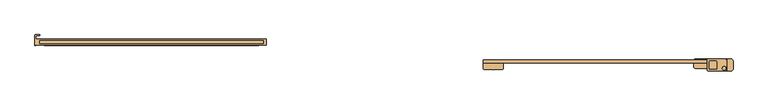
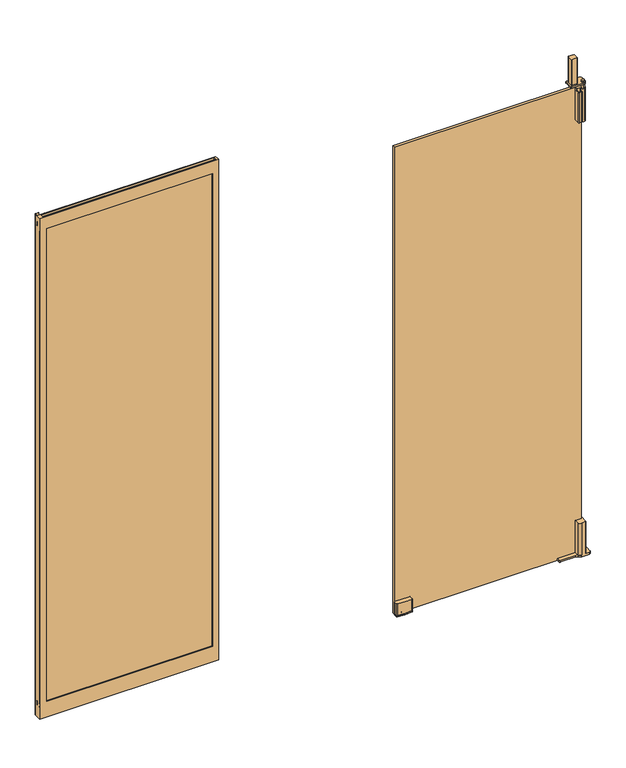
"""IFC4 building model written with IfcOpenShell, lengths in millimetres: door geometry, Otomatik Kapı-Çift Kanat : Otomatik Kapı - Çift Kanat - 150-220."""

from ifc_helpers import new_model, si_unit, frame, origin, origin_with_axes, place, context, project, spatial, polyline, circle_curve, outline, extrude, source, transform, mapped, element, save
from ifc_brep_helpers import plane_surface, cylinder_surface, revolved_surface, advanced_brep


def door_5e92e189(model_context):
    return source(origin(), model_context, "Body", "SolidModel", [
        advanced_brep(
        [(-756.7, 35.2330503, 8.0000212), (-753.7330503, 38.2, 8.0000212), (-741.69925, 38.2, 8.0000212), (-741.69925, 36.2, 8.0000212), (-753.6861454, 36.2, 8.0000212), (-754.7, 35.1861454, 8.0000212), (-754.7, 23.7, 8.0000212), (-2.5, 23.6999918, 8.0000212), (-2.5, 3.7, 8.0000212), (-756.7, 3.7, 8.0000212), (-741.69925, 10.2025832, 8.0000212), (-12.4985, 10.2025832, 8.0000212), (-12.4985, 17.1998167, 8.0000212), (-741.69925, 17.1998167, 8.0000212), (-754.7, 23.7, 2241.0), (-754.7, 35.1861454, 2241.0), (-753.6861454, 36.2, 2241.0), (-741.69925, 36.2, 2241.0), (-741.69925, 38.2, 2241.0), (-753.7330503, 38.2, 2241.0), (-756.7, 35.2330503, 2241.0), (-756.7, 3.7, 2241.0), (-2.5, 3.7, 2241.0), (-2.5, 23.7, 2241.0), (-741.69925, 18.701, 2241.0), (-12.4985, 18.701, 2241.0), (-12.4985, 8.699, 2241.0), (-741.69925, 8.699, 2241.0), (-756.7, 3.7, 78.000055), (-756.7, 5.7, 78.000055), (-756.7, 5.7, 62.9982446), (-756.7, 6.760542, 62.9982446), (-756.7, 6.760542, 2201.0007973), (-756.7, 5.7, 2201.0007973), (-756.7, 5.7, 2186.0007973), (-756.7, 3.7, 2186.0007973), (-726.6862373, 23.7, 2186.0004744), (-726.6862373, 21.7006279, 2186.0004744), (-726.6862373, 21.7006279, 77.9999799), (-726.6862373, 23.7, 77.9999799), (-741.69925, 21.7006279, 2201.0007973), (-741.69925, 21.7006279, 62.9982446), (-12.4985, 21.7006279, 62.9982446), (-12.4985, 21.7006279, 2201.0007973), (-27.4985, 21.7006279, 2186.0004744), (-27.4985, 21.7006279, 77.9999799), (-741.69925, 17.1998167, 33.4998483), (-741.69925, 10.2025832, 33.4998483), (-741.69925, 8.699, 2232.5), (-741.69925, 18.701, 2232.5), (-741.69925, 5.7, 2201.0007973), (-741.69925, 5.7, 62.9982446), (-756.5103756, 5.7, 78.000055), (-756.5103756, 5.7, 62.9982446), (-756.5103756, 5.7, 2201.0007973), (-756.5103756, 5.7, 2186.0007973), (-12.4985, 5.7, 2201.0007973), (-12.4985, 5.7, 62.9982446), (-726.6985, 5.7, 2186.0007973), (-726.6985, 5.7, 78.000055), (-27.4985, 5.7, 78.000055), (-27.4985, 5.7, 2186.0007973), (-726.6985, 3.7, 2186.0007973), (-726.6985, 3.7, 78.000055), (-753.639458, 3.7, 2186.0007973), (-753.639458, 3.7, 78.000055), (-27.4985, 3.7, 2186.0007973), (-27.4985, 3.7, 78.000055), (-27.4985, 23.7, 77.9999799), (-27.4985, 23.7, 2186.0004744), (-12.4985, 8.699, 2232.5), (-12.4985, 18.701, 2232.5), (-12.4985, 17.1998167, 33.4998483), (-12.4985, 10.2025832, 33.4998483)],
        [
            (0, 1, circle_curve(frame((-753.7330503, 35.2330503, 8.0000212), z_axis=(0.0, 0.0, -1.0), x_axis=(-1.0, 0.0, 0.0)), 2.9669497)),
            (1, 2),
            (2, 3),
            (3, 4),
            (4, 5, circle_curve(frame((-753.6861454, 35.1861454, 8.0000212), z_axis=(0.0, 0.0, 1.0), x_axis=(-1.0, 0.0, 0.0)), 1.0138546)),
            (5, 6),
            (6, 7),
            (7, 8),
            (8, 9),
            (9, 0),
            (10, 11),
            (11, 12),
            (12, 13),
            (13, 10),
            (14, 15),
            (15, 16, circle_curve(frame((-753.6861454, 35.1861454, 2241.0), z_axis=(0.0, 0.0, -1.0), x_axis=(-1.0, 0.0, 0.0)), 1.0138546)),
            (16, 17),
            (17, 18),
            (18, 19),
            (19, 20, circle_curve(frame((-753.7330503, 35.2330503, 2241.0), z_axis=(0.0, 0.0, 1.0), x_axis=(-1.0, 0.0, 0.0)), 2.9669497)),
            (20, 21),
            (21, 22),
            (22, 23),
            (23, 14),
            (24, 25),
            (25, 26),
            (26, 27),
            (27, 24),
            (20, 0),
            (9, 28),
            (28, 29),
            (29, 30),
            (30, 31),
            (31, 32),
            (32, 33),
            (33, 34),
            (34, 35),
            (35, 21),
            (1, 19),
            (18, 2),
            (17, 3),
            (36, 37),
            (37, 38),
            (38, 39),
            (39, 36),
            (40, 41),
            (41, 42),
            (42, 43),
            (43, 40),
            (37, 44),
            (44, 45),
            (45, 38),
            (13, 46),
            (46, 47),
            (47, 10),
            (27, 48),
            (48, 49),
            (49, 24),
            (40, 50),
            (50, 51),
            (51, 41),
            (29, 52),
            (52, 53),
            (53, 30),
            (33, 54),
            (54, 55),
            (55, 34),
            (50, 56),
            (56, 57),
            (57, 51),
            (58, 59),
            (59, 60),
            (60, 61),
            (61, 58),
            (58, 62),
            (62, 63),
            (63, 59),
            (35, 64),
            (64, 65),
            (65, 28),
            (8, 22),
            (62, 66),
            (66, 67),
            (67, 63),
            (23, 7),
            (6, 14),
            (39, 68),
            (68, 69),
            (69, 36),
            (16, 4),
            (5, 15),
            (54, 32, circle_curve(frame((-753.639458, 6.760542, 2201.0007973), z_axis=(0.0, 0.0, -1.0), x_axis=(-1.0, 0.0, 0.0)), 3.060542)),
            (31, 53, circle_curve(frame((-753.639458, 6.760542, 62.9982446), z_axis=(0.0, 0.0, 1.0), x_axis=(-1.0, 0.0, 0.0)), 3.060542)),
            (52, 65, circle_curve(frame((-753.639458, 6.760542, 78.000055), z_axis=(0.0, 0.0, 1.0), x_axis=(-1.0, 0.0, 0.0)), 3.060542)),
            (64, 55, circle_curve(frame((-753.639458, 6.760542, 2186.0007973), z_axis=(0.0, 0.0, -1.0), x_axis=(-1.0, 0.0, 0.0)), 3.060542)),
            (26, 70),
            (70, 48),
            (70, 71),
            (71, 49),
            (71, 25),
            (69, 44),
            (43, 56),
            (61, 66),
            (67, 60),
            (57, 42),
            (45, 68),
            (12, 72),
            (72, 46),
            (72, 73),
            (73, 47),
            (73, 11),
        ],
        [
            plane_surface(frame((-756.7, 23.7, 8.0000212), z_axis=(0.0, 0.0, -1.0), x_axis=(0.0, -1.0, 0.0))),
            plane_surface(frame((-756.7, 23.7, 2241.0), z_axis=(0.0, 0.0, 1.0), x_axis=(0.0, -1.0, 0.0))),
            plane_surface(frame((-756.7, 6.760542, 8.0000212), z_axis=(-1.0, 0.0, 0.0), x_axis=(0.0, 0.0, 1.0))),
            plane_surface(frame((-753.7330503, 38.2, 8.0000212), z_axis=(0.0, 1.0, 0.0), x_axis=(0.0, 0.0, 1.0))),
            plane_surface(frame((-741.69925, 38.2, 8.0000212), z_axis=(1.0, 0.0, 0.0), x_axis=(0.0, 0.0, 1.0))),
            plane_surface(frame((-726.6862373, 23.7, 8.0000212), z_axis=(1.0, 0.0, 0.0), x_axis=(0.0, 0.0, 1.0))),
            plane_surface(frame((-726.6862373, 21.7006279, 8.0000212), z_axis=(0.0, -1.0, 0.0), x_axis=(0.0, 0.0, 1.0))),
            plane_surface(frame((-741.69925, 21.7006279, 8.0000212), z_axis=(1.0, 0.0, 0.0), x_axis=(0.0, 0.0, 1.0))),
            plane_surface(frame((-741.69925, 5.7, 8.0000212), z_axis=(0.0, 1.0, 0.0), x_axis=(0.0, 0.0, 1.0))),
            plane_surface(frame((-726.6985, 5.7, 8.0000212), z_axis=(1.0, 0.0, 0.0), x_axis=(0.0, 0.0, 1.0))),
            plane_surface(frame((-726.6985, 3.7, 8.0000212), z_axis=(0.0, -1.0, 0.0), x_axis=(0.0, 0.0, 1.0))),
            plane_surface(frame((-754.7, 23.7, 8.0000212), z_axis=(0.0, 1.0, 0.0), x_axis=(0.0, 0.0, 1.0))),
            plane_surface(frame((-741.69925, 36.2, 8.0000212), z_axis=(0.0, -1.0, 0.0), x_axis=(0.0, 0.0, 1.0))),
            plane_surface(frame((-754.7, 35.1861454, 8.0000212), z_axis=(1.0, 0.0, 0.0), x_axis=(0.0, 0.0, 1.0))),
            cylinder_surface(frame((-753.639458, 6.760542, 8.0000212), z_axis=(0.0, 0.0, -1.0), x_axis=(-1.0, 0.0, 0.0)), 3.060542),
            cylinder_surface(frame((-753.7330503, 35.2330503, 8.0000212), z_axis=(0.0, 0.0, -1.0), x_axis=(-1.0, 0.0, 0.0)), 2.9669497),
            revolved_surface(polyline([(-754.6999999999999, 35.1861454, 2241.0), (-754.6999999999999, 35.1861454, 8.0000212)]), (-753.6861454, 35.1861454, 8.0000212), (0.0, 0.0, 1.0)),
            plane_surface(frame((-2.5, 23.7, 2241.0), z_axis=(1.0, 0.0, 0.0), x_axis=(0.0, -1.0, 0.0))),
            plane_surface(frame((-756.7, 8.699, 2241.0), z_axis=(0.0, 1.0, 0.0), x_axis=(1.0, 0.0, 0.0))),
            plane_surface(frame((-756.7, 8.699, 2232.5), z_axis=(0.0, 0.0, 1.0), x_axis=(1.0, 0.0, 0.0))),
            plane_surface(frame((-756.7, 18.701, 2232.5), z_axis=(0.0, -1.0, 0.0), x_axis=(1.0, 0.0, 0.0))),
            plane_surface(frame((-756.7, 23.7, 2186.0004744), z_axis=(0.0, 0.0, -1.0), x_axis=(1.0, 0.0, 0.0))),
            plane_surface(frame((-756.7, 21.7, 2201.0007973), z_axis=(0.0, 0.0, -1.0), x_axis=(1.0, 0.0, 0.0))),
            plane_surface(frame((-756.7, 5.7, 2186.0007973), z_axis=(0.0, 0.0, -1.0), x_axis=(1.0, 0.0, 0.0))),
            plane_surface(frame((-756.7, 3.7, 78.000055), z_axis=(0.0, 0.0, 1.0), x_axis=(1.0, 0.0, 0.0))),
            plane_surface(frame((-756.7, 5.7, 62.9982446), z_axis=(0.0, 0.0, 1.0), x_axis=(1.0, 0.0, 0.0))),
            plane_surface(frame((-756.7, 21.6999777, 77.9999799), z_axis=(0.0, 0.0, 1.0), x_axis=(1.0, 0.0, 0.0))),
            plane_surface(frame((-756.7, 17.1998167, 8.0000212), z_axis=(0.0, -1.0, 0.0), x_axis=(1.0, 0.0, 0.0))),
            plane_surface(frame((-756.7, 17.1998167, 33.4998483), z_axis=(0.0, 0.0, -1.0), x_axis=(1.0, 0.0, 0.0))),
            plane_surface(frame((-756.7, 10.2025832, 33.4998483), z_axis=(0.0, 1.0, 0.0), x_axis=(1.0, 0.0, 0.0))),
            plane_surface(frame((-27.4985, 3.7, 8.0000212), z_axis=(-1.0, 0.0, 0.0), x_axis=(0.0, 0.0, 1.0))),
            plane_surface(frame((-12.4985, 5.7, 8.0000212), z_axis=(-1.0, 0.0, 0.0), x_axis=(0.0, 0.0, 1.0))),
            plane_surface(frame((-27.4985, 21.7, 8.0000212), z_axis=(-1.0, 0.0, 0.0), x_axis=(0.0, 0.0, 1.0))),
        ],
        [
            (0, [[1, 2, 3, 4, 5, 6, 7, 8, 9, 10], [11, 12, 13, 14]]),
            (1, [[15, 16, 17, 18, 19, 20, 21, 22, 23, 24], [25, 26, 27, 28]]),
            (2, [[29, -10, 30, 31, 32, 33, 34, 35, 36, 37, 38, -21]]),
            (3, [[-2, 39, -19, 40]]),
            (4, [[-3, -40, -18, 41]]),
            (5, [[42, 43, 44, 45]]),
            (6, [[46, 47, 48, 49], [-43, 50, 51, 52]]),
            (7, [[-14, 53, 54, 55]]),
            (7, [[-28, 56, 57, 58]]),
            (7, [[59, 60, 61, -46]]),
            (8, [[-32, 62, 63, 64]]),
            (8, [[-36, 65, 66, 67]]),
            (8, [[-60, 68, 69, 70], [71, 72, 73, 74]]),
            (9, [[75, 76, 77, -71]]),
            (10, [[-22, -38, 78, 79, 80, -30, -9, 81], [82, 83, 84, -76]]),
            (11, [[-24, 85, -7, 86], [87, 88, 89, -45]]),
            (12, [[-4, -41, -17, 90]]),
            (13, [[-6, 91, -15, -86]]),
            (14, [[92, -34, 93, -63, 94, -79, 95, -66]]),
            (15, [[-1, -29, -20, -39]]),
            (16, [[-5, -90, -16, -91]]),
            (17, [[-81, -8, -85, -23]]),
            (18, [[-56, -27, 96, 97]]),
            (19, [[-57, -97, 98, 99]]),
            (20, [[-58, -99, 100, -25]]),
            (21, [[-42, -89, 101, -50]]),
            (22, [[-35, -92, -65]]),
            (22, [[-68, -59, -49, 102]]),
            (23, [[-37, -67, -95, -78]]),
            (23, [[-75, -74, 103, -82]]),
            (24, [[-31, -80, -94, -62]]),
            (24, [[-77, -84, 104, -72]]),
            (25, [[-33, -64, -93]]),
            (25, [[-47, -61, -70, 105]]),
            (26, [[-44, -52, 106, -87]]),
            (27, [[-53, -13, 107, 108]]),
            (28, [[-54, -108, 109, 110]]),
            (29, [[-55, -110, 111, -11]]),
            (30, [[-73, -104, -83, -103]]),
            (31, [[-12, -111, -109, -107]]),
            (31, [[-26, -100, -98, -96]]),
            (31, [[-69, -102, -48, -105]]),
            (32, [[-88, -106, -51, -101]]),
        ],
    ),
        extrude(outline(polyline([(-14.9985, 20.6999853), (-14.9985, 10.7006304), (-738.2, 10.7006304), (-738.2, 20.6999853), (-14.9985, 20.6999853)])), frame((0.0, 0.0, 65.4907153), z_axis=(0.0, 0.0, 1.0), x_axis=(1.0, 0.0, 0.0)), (0.0, 0.0, 1.0), 2133.010082),
        extrude(outline(polyline([(20.6999607, 2198.9584681), (20.6999633, 2215.4578872), (21.6999632, 2215.4578872), (21.6999608, 2200.1996761), (23.2999608, 2200.1994116), (23.2999608, 2199.1856312), (20.6999607, 2198.9584681)])), frame((-756.7, 0.0, 0.0), z_axis=(1.0, 0.0, 0.0), x_axis=(0.0, 1.0, 0.0)), (0.0, 0.0, 1.0), 754.2),
        extrude(outline(polyline([(20.6999853, 79.2411881), (23.2999854, 79.0140251), (23.2999854, 78.0002446), (21.6999855, 77.9999802), (21.6999855, 62.7412326), (20.6999879, 62.7417691), (20.6999853, 79.2411881)])), frame((-756.7, 0.0, 0.0), z_axis=(1.0, 0.0, 0.0), x_axis=(0.0, 1.0, 0.0)), (0.0, 0.0, 1.0), 754.2),
        extrude(outline(polyline([(-737.3860852, 21.7000002), (-726.7, 21.7000002), (-726.7, 23.3000002), (-725.585912, 23.3000002), (-725.2906874, 20.49978), (-737.3860852, 20.49978), (-737.3860852, 21.7000002)])), frame((0.0, 0.0, 8.0000212), z_axis=(0.0, 0.0, 1.0), x_axis=(1.0, 0.0, 0.0)), (0.0, 0.0, 1.0), 2232.9999788),
        advanced_brep(
        [(1467.3535836, -45.0, 150.5), (1493.0, -45.0, 150.5), (1493.0, -54.9832441, 150.5), (1468.0, -54.9832441, 150.5), (1468.0, -73.2159914, 150.5), (1480.406782, -80.0, 150.5), (1498.2162961, -80.0, 150.5), (1500.0, -78.2162961, 150.5), (1500.0, -42.932554, 150.5), (1498.067446, -41.0, 150.5), (1469.2861376, -41.0, 150.5), (1467.3535836, -42.932554, 150.5), (1471.9265924, -76.964766, 8.0), (1468.0, -73.2159914, 8.0), (1470.1692976, -75.2261826, 8.0), (1467.3535836, -45.0, 8.0), (1493.0, -45.0, 8.0), (1493.0, -54.9832441, 8.0), (1468.0, -54.9832441, 8.0), (1480.406782, -80.0, 8.0), (1480.406782, -80.0, 0.0), (1512.8478933, -80.0, 0.0), (1512.8478933, -80.0, 8.0), (1498.2162961, -80.0, 8.0), (1500.0, -78.2162961, 8.0), (1500.0, -42.932554, 8.0), (1498.067446, -41.0, 8.0), (1512.9502869, -41.0, 8.0), (1512.9502869, -41.0, 0.0), (1397.0062198, -41.0, 0.0), (1397.0062198, -41.0, 8.0), (1469.2861376, -41.0, 8.0), (1467.3535836, -42.932554, 8.0), (1520.0062198, -48.0559329, 0.0), (1520.0062198, -72.8416735, 0.0), (1470.1692976, -75.2261826, 0.0), (1461.1062198, -71.0, 0.0), (1397.0062198, -71.0, 0.0), (1392.0062198, -66.0, 0.0), (1392.0062198, -46.0, 0.0), (1520.0062198, -72.8416735, 8.0), (1520.0062198, -48.0559329, 8.0), (1392.0062198, -46.0, 8.0), (1392.0062198, -66.0, 8.0), (1397.0062198, -71.0, 8.0), (1461.1062198, -71.0, 8.0)],
        [
            (0, 1),
            (1, 2),
            (2, 3),
            (3, 4),
            (4, 5, circle_curve(frame((1481.829294, -62.6615339, 150.5), z_axis=(0.0, 0.0, 1.0), x_axis=(-1.0, 0.0, 0.0)), 17.3967223)),
            (5, 6),
            (6, 7, circle_curve(frame((1498.2162961, -78.2162961, 150.5), z_axis=(0.0, 0.0, 1.0), x_axis=(-1.0, 0.0, 0.0)), 1.7837039)),
            (7, 8),
            (8, 9, circle_curve(frame((1498.067446, -42.932554, 150.5), z_axis=(0.0, 0.0, 1.0), x_axis=(-1.0, 0.0, 0.0)), 1.932554)),
            (9, 10),
            (10, 11, circle_curve(frame((1469.2861376, -42.932554, 150.5), z_axis=(0.0, 0.0, 1.0), x_axis=(-1.0, 0.0, 0.0)), 1.932554)),
            (11, 0),
            (12, 13, circle_curve(frame((1481.829294, -62.6615339, 8.0), z_axis=(0.0, 0.0, -1.0), x_axis=(-1.0, 0.0, 0.0)), 17.3967223)),
            (13, 14, circle_curve(frame((1461.1062198, -82.8310079, 8.0), z_axis=(0.0, 0.0, -1.0), x_axis=(-1.0, 0.0, 0.0)), 11.8310079)),
            (14, 12, circle_curve(frame((1480.406782, -66.6359132, 8.0), z_axis=(0.0, 0.0, 1.0), x_axis=(-1.0, 0.0, 0.0)), 13.3640868)),
            (0, 15),
            (15, 16),
            (16, 1),
            (16, 17),
            (17, 2),
            (17, 18),
            (18, 3),
            (18, 13),
            (13, 4),
            (12, 19, circle_curve(frame((1481.829294, -62.6615339, 8.0), z_axis=(0.0, 0.0, 1.0), x_axis=(-1.0, 0.0, 0.0)), 17.3967223)),
            (19, 5),
            (19, 20),
            (20, 21),
            (21, 22),
            (22, 23),
            (23, 6),
            (23, 24, circle_curve(frame((1498.2162961, -78.2162961, 8.0), z_axis=(0.0, 0.0, 1.0), x_axis=(-1.0, 0.0, 0.0)), 1.7837039)),
            (24, 7),
            (24, 25),
            (25, 8),
            (25, 26, circle_curve(frame((1498.067446, -42.932554, 8.0), z_axis=(0.0, 0.0, 1.0), x_axis=(-1.0, 0.0, 0.0)), 1.932554)),
            (26, 9),
            (26, 27),
            (27, 28),
            (28, 29),
            (29, 30),
            (30, 31),
            (31, 10),
            (31, 32, circle_curve(frame((1469.2861376, -42.932554, 8.0), z_axis=(0.0, 0.0, 1.0), x_axis=(-1.0, 0.0, 0.0)), 1.932554)),
            (32, 11),
            (32, 15),
            (28, 33, circle_curve(frame((1512.9502869, -48.0559329, 0.0), z_axis=(0.0, 0.0, -1.0), x_axis=(-1.0, 0.0, 0.0)), 7.0559329)),
            (33, 34),
            (34, 21, circle_curve(frame((1512.8478933, -72.8416735, 0.0), z_axis=(0.0, 0.0, -1.0), x_axis=(-1.0, 0.0, 0.0)), 7.1583265)),
            (20, 35, circle_curve(frame((1480.406782, -66.6359132, 0.0), z_axis=(0.0, 0.0, -1.0), x_axis=(-1.0, 0.0, 0.0)), 13.3640868)),
            (35, 36, circle_curve(frame((1461.1062198, -82.8310079, 0.0), z_axis=(0.0, 0.0, 1.0), x_axis=(-1.0, 0.0, 0.0)), 11.8310079)),
            (36, 37),
            (37, 38, circle_curve(frame((1397.0062198, -66.0, 0.0), z_axis=(0.0, 0.0, -1.0), x_axis=(-1.0, 0.0, 0.0)), 5.0)),
            (38, 39),
            (39, 29, circle_curve(frame((1397.0062198, -46.0, 0.0), z_axis=(0.0, 0.0, -1.0), x_axis=(-1.0, 0.0, 0.0)), 5.0)),
            (12, 19, circle_curve(frame((1480.406782, -66.6359132, 8.0), z_axis=(0.0, 0.0, 1.0), x_axis=(-1.0, 0.0, 0.0)), 13.3640868)),
            (22, 40, circle_curve(frame((1512.8478933, -72.8416735, 8.0), z_axis=(0.0, 0.0, 1.0), x_axis=(-1.0, 0.0, 0.0)), 7.1583265)),
            (40, 41),
            (41, 27, circle_curve(frame((1512.9502869, -48.0559329, 8.0), z_axis=(0.0, 0.0, 1.0), x_axis=(-1.0, 0.0, 0.0)), 7.0559329)),
            (30, 42, circle_curve(frame((1397.0062198, -46.0, 8.0), z_axis=(0.0, 0.0, 1.0), x_axis=(-1.0, 0.0, 0.0)), 5.0)),
            (42, 43),
            (43, 44, circle_curve(frame((1397.0062198, -66.0, 8.0), z_axis=(0.0, 0.0, 1.0), x_axis=(-1.0, 0.0, 0.0)), 5.0)),
            (44, 45),
            (45, 13, circle_curve(frame((1461.1062198, -82.8310079, 8.0), z_axis=(0.0, 0.0, -1.0), x_axis=(-1.0, 0.0, 0.0)), 11.8310079)),
            (41, 33),
            (40, 34),
            (14, 35),
            (45, 36),
            (44, 37),
            (43, 38),
            (42, 39),
        ],
        [
            plane_surface(frame((1520.0062198, -41.0, 150.5), z_axis=(0.0, 0.0, 1.0), x_axis=(0.0, 1.0, 0.0))),
            plane_surface(frame((1520.0062198, -41.0, 8.0), z_axis=(0.0, 0.0, -1.0), x_axis=(0.0, 1.0, 0.0))),
            plane_surface(frame((1467.3535836, -45.0, 150.5), z_axis=(0.0, -1.0, 0.0), x_axis=(0.0, 0.0, -1.0))),
            plane_surface(frame((1493.0, -45.0, 150.5), z_axis=(-1.0, 0.0, 0.0), x_axis=(0.0, 0.0, -1.0))),
            plane_surface(frame((1493.0, -54.9832441, 150.5), z_axis=(0.0, 1.0, 0.0), x_axis=(0.0, 0.0, -1.0))),
            plane_surface(frame((1468.0, -54.9832441, 150.5), z_axis=(-1.0, 0.0, 0.0), x_axis=(0.0, 0.0, -1.0))),
            cylinder_surface(frame((1481.829294, -62.6615339, 150.5), z_axis=(0.0, 0.0, 1.0), x_axis=(-1.0, 0.0, 0.0)), 17.3967223),
            plane_surface(frame((1480.406782, -80.0, 150.5), z_axis=(0.0, -1.0, 0.0), x_axis=(0.0, 0.0, -1.0))),
            cylinder_surface(frame((1498.2162961, -78.2162961, 150.5), z_axis=(0.0, 0.0, 1.0), x_axis=(-1.0, 0.0, 0.0)), 1.7837039),
            plane_surface(frame((1500.0, -78.2162961, 150.5), z_axis=(1.0, 0.0, 0.0), x_axis=(0.0, 0.0, -1.0))),
            cylinder_surface(frame((1498.067446, -42.932554, 150.5), z_axis=(0.0, 0.0, 1.0), x_axis=(-1.0, 0.0, 0.0)), 1.932554),
            plane_surface(frame((1498.067446, -41.0, 150.5), z_axis=(0.0, 1.0, 0.0), x_axis=(0.0, 0.0, -1.0))),
            cylinder_surface(frame((1469.2861376, -42.932554, 150.5), z_axis=(0.0, 0.0, 1.0), x_axis=(-1.0, 0.0, 0.0)), 1.932554),
            plane_surface(frame((1467.3535836, -42.932554, 150.5), z_axis=(-1.0, 0.0, 0.0), x_axis=(0.0, 0.0, -1.0))),
            plane_surface(frame((1520.0062198, -41.0, 0.0), z_axis=(0.0, 0.0, -1.0), x_axis=(0.0, 1.0, 0.0))),
            plane_surface(frame((1520.0062198, -41.0, 8.0), z_axis=(0.0, 0.0, 1.0), x_axis=(0.0, 1.0, 0.0))),
            cylinder_surface(frame((1512.9502869, -48.0559329, 0.0), z_axis=(0.0, 0.0, -1.0), x_axis=(-1.0, 0.0, 0.0)), 7.0559329),
            plane_surface(frame((1520.0062198, -48.0559329, 0.0), z_axis=(1.0, 0.0, 0.0), x_axis=(0.0, 0.0, 1.0))),
            cylinder_surface(frame((1512.8478933, -72.8416735, 0.0), z_axis=(0.0, 0.0, -1.0), x_axis=(-1.0, 0.0, 0.0)), 7.1583265),
            cylinder_surface(frame((1480.406782, -66.6359132, 0.0), z_axis=(0.0, 0.0, -1.0), x_axis=(-1.0, 0.0, 0.0)), 13.3640868),
            revolved_surface(polyline([(1449.2752119, -82.8310079, 8.0), (1449.2752119, -82.8310079, 0.0)]), (1461.1062198, -82.8310079, 0.0), (0.0, 0.0, 1.0)),
            plane_surface(frame((1461.1062198, -71.0, 0.0), z_axis=(0.0, -1.0, 0.0), x_axis=(0.0, 0.0, 1.0))),
            cylinder_surface(frame((1397.0062198, -66.0, 0.0), z_axis=(0.0, 0.0, -1.0), x_axis=(-1.0, 0.0, 0.0)), 5.0),
            plane_surface(frame((1392.0062198, -66.0, 0.0), z_axis=(-1.0, 0.0, 0.0), x_axis=(0.0, 0.0, 1.0))),
            cylinder_surface(frame((1397.0062198, -46.0, 0.0), z_axis=(0.0, 0.0, -1.0), x_axis=(-1.0, 0.0, 0.0)), 5.0),
        ],
        [
            (0, [[1, 2, 3, 4, 5, 6, 7, 8, 9, 10, 11, 12]]),
            (1, [[13, 14, 15]]),
            (2, [[-1, 16, 17, 18]]),
            (3, [[-2, -18, 19, 20]]),
            (4, [[-3, -20, 21, 22]]),
            (5, [[-4, -22, 23, 24]]),
            (6, [[-5, -24, -13, 25, 26]]),
            (7, [[-6, -26, 27, 28, 29, 30, 31]]),
            (8, [[-7, -31, 32, 33]]),
            (9, [[-8, -33, 34, 35]]),
            (10, [[-9, -35, 36, 37]]),
            (11, [[-10, -37, 38, 39, 40, 41, 42, 43]]),
            (12, [[-11, -43, 44, 45]]),
            (13, [[-12, -45, 46, -16]]),
            (14, [[-40, 47, 48, 49, -28, 50, 51, 52, 53, 54, 55]]),
            (15, [[56, -25]]),
            (15, [[57, 58, 59, -38, -36, -34, -32, -30]]),
            (15, [[60, 61, 62, 63, 64, -23, -21, -19, -17, -46, -44, -42]]),
            (16, [[-47, -39, -59, 65]]),
            (17, [[-48, -65, -58, 66]]),
            (18, [[-49, -66, -57, -29]]),
            (19, [[-50, -27, -56, -15, 67]]),
            (20, [[-51, -67, -14, -64, 68]]),
            (21, [[-52, -68, -63, 69]]),
            (22, [[-53, -69, -62, 70]]),
            (23, [[-54, -70, -61, 71]]),
            (24, [[-55, -71, -60, -41]]),
        ],
    ),
        advanced_brep(
        [(1465.150075, -48.2790947, 2225.0), (1443.8206454, -48.2790947, 2225.0), (1441.9853602, -50.1143799, 2225.0), (1441.9853602, -71.4438095, 2225.0), (1443.8206454, -73.2790947, 2225.0), (1465.150075, -73.2790947, 2225.0), (1466.9853602, -71.4438095, 2225.0), (1466.9853602, -50.1143799, 2225.0), (1465.150075, -48.2790947, 2110.0), (1443.8206454, -48.2790947, 2110.0), (1441.9853602, -50.1143799, 2110.0), (1441.9853602, -71.4438095, 2110.0), (1443.8206454, -73.2790947, 2110.0), (1465.150075, -73.2790947, 2110.0), (1466.9853602, -71.4438095, 2110.0), (1466.9853602, -50.1143799, 2110.0), (1439.0026222, -41.0, 2110.0), (1436.0, -44.0026222, 2110.0), (1436.0, -77.6784243, 2110.0), (1439.3215757, -81.0, 2110.0), (1491.0, -81.0, 2110.0), (1500.0, -72.0, 2110.0), (1500.0, -49.8288404, 2110.0), (1491.1711596, -41.0, 2110.0), (1491.0, -77.9, 2110.0), (1491.0, -66.1, 2110.0), (1439.0026222, -41.0, 2104.0), (1491.1711596, -41.0, 2104.0), (1500.0, -49.8288404, 2104.0), (1500.0, -72.0, 2104.0), (1491.0, -81.0, 2104.0), (1439.3215757, -81.0, 2104.0), (1436.0, -77.6784243, 2104.0), (1436.0, -44.0026222, 2104.0), (1491.0, -66.1, 2104.0), (1491.0, -77.9, 2104.0), (1500.0, -72.0, 1938.2), (1484.4524153, -78.1748793, 1938.2), (1480.4177248, -81.0, 1938.2), (1471.1, -81.0, 1938.2), (1468.0, -77.9, 1938.2), (1468.0, -55.1, 1938.2), (1492.8, -55.1, 1938.2), (1492.8, -45.1, 1938.2), (1468.0, -45.1, 1938.2), (1468.0, -42.3259879, 1938.2), (1469.3259879, -41.0, 1938.2), (1498.7883994, -41.0, 1938.2), (1500.0, -42.2116006, 1938.2), (1480.2256421, -66.1, 1938.2), (1471.1, -66.1, 1938.2), (1471.1, -76.9112221, 1938.2), (1472.0887779, -77.9, 1938.2), (1480.1735897, -77.9, 1938.2), (1481.9491878, -75.7274684, 1938.2), (1482.0, -67.8743579, 1938.2), (1491.0, -66.1, 1938.2), (1491.0, -77.9, 1938.2), (1500.0, -72.0, 2083.2), (1500.0, -42.2116006, 2083.2), (1498.7883994, -41.0, 2083.2), (1469.3259879, -41.0, 2083.2), (1468.0, -42.3259879, 2083.2), (1468.0, -45.1, 2083.2), (1492.8, -45.1, 2083.2), (1492.8, -55.1, 2083.2), (1468.0, -55.1, 2083.2), (1468.0, -64.9220198, 2083.2), (1469.1779802, -66.1, 2083.2), (1480.2256421, -66.1, 2083.2), (1482.0, -67.8743579, 2083.2), (1482.0, -72.0, 2083.2), (1491.0, -77.9, 2083.2), (1491.0, -66.1, 2083.2), (1468.0, -77.9, 2073.2), (1468.0, -64.9220198, 2073.2), (1469.1779802, -66.1, 2073.2), (1471.1, -66.1, 2073.2), (1482.0, -75.7274684, 2073.2), (1482.0, -72.0, 2073.2), (1484.4524153, -78.1748793, 2073.2), (1491.0, -77.9, 2083.2), (1491.0, -66.1, 2083.2), (1471.1, -81.0, 2073.2), (1480.4177248, -81.0, 2073.2), (1480.1735897, -77.9, 2073.2), (1472.0887779, -77.9, 2073.2), (1471.1, -76.9112221, 2073.2), (1491.0, -66.1, 2116.5286826), (1491.0, -77.9, 2116.5286826)],
        [
            (0, 1),
            (1, 2, circle_curve(frame((1443.8206454, -50.1143799, 2225.0), z_axis=(0.0, 0.0, 1.0), x_axis=(0.0, -1.0, 0.0)), 1.8352852)),
            (2, 3),
            (3, 4, circle_curve(frame((1443.8206454, -71.4438095, 2225.0), z_axis=(0.0, 0.0, 1.0), x_axis=(0.0, 1.0, 0.0)), 1.8352852)),
            (4, 5),
            (5, 6, circle_curve(frame((1465.150075, -71.4438095, 2225.0), z_axis=(0.0, 0.0, 1.0), x_axis=(0.0, 1.0, 0.0)), 1.8352852)),
            (6, 7),
            (7, 0, circle_curve(frame((1465.150075, -50.1143799, 2225.0), z_axis=(0.0, 0.0, 1.0), x_axis=(0.0, -1.0, 0.0)), 1.8352852)),
            (0, 8),
            (8, 9),
            (9, 1),
            (9, 10, circle_curve(frame((1443.8206454, -50.1143799, 2110.0), z_axis=(0.0, 0.0, 1.0), x_axis=(0.0, -1.0, 0.0)), 1.8352852)),
            (10, 2),
            (10, 11),
            (11, 3),
            (11, 12, circle_curve(frame((1443.8206454, -71.4438095, 2110.0), z_axis=(0.0, 0.0, 1.0), x_axis=(0.0, 1.0, 0.0)), 1.8352852)),
            (12, 4),
            (12, 13),
            (13, 5),
            (13, 14, circle_curve(frame((1465.150075, -71.4438095, 2110.0), z_axis=(0.0, 0.0, 1.0), x_axis=(0.0, 1.0, 0.0)), 1.8352852)),
            (14, 6),
            (14, 15),
            (15, 7),
            (15, 8, circle_curve(frame((1465.150075, -50.1143799, 2110.0), z_axis=(0.0, 0.0, 1.0), x_axis=(0.0, -1.0, 0.0)), 1.8352852)),
            (16, 17, circle_curve(frame((1439.0026222, -44.0026222, 2110.0), z_axis=(0.0, 0.0, 1.0), x_axis=(0.0, -1.0, 0.0)), 3.0026222)),
            (17, 18),
            (18, 19, circle_curve(frame((1439.3215757, -77.6784243, 2110.0), z_axis=(0.0, 0.0, 1.0), x_axis=(0.0, -1.0, 0.0)), 3.3215757)),
            (19, 20),
            (20, 21, circle_curve(frame((1491.0, -72.0, 2110.0), z_axis=(0.0, 0.0, 1.0), x_axis=(0.0, -1.0, 0.0)), 9.0)),
            (21, 22),
            (22, 23, circle_curve(frame((1491.1711596, -49.8288404, 2110.0), z_axis=(0.0, 0.0, 1.0), x_axis=(0.0, -1.0, 0.0)), 8.8288404)),
            (23, 16),
            (24, 25, circle_curve(frame((1491.0, -72.0, 2110.0), z_axis=(0.0, 0.0, -1.0), x_axis=(0.0, -1.0, 0.0)), 5.9)),
            (25, 24, circle_curve(frame((1491.0, -72.0, 2110.0), z_axis=(0.0, 0.0, -1.0), x_axis=(0.0, -1.0, 0.0)), 5.9)),
            (26, 27),
            (27, 28, circle_curve(frame((1491.1711596, -49.8288404, 2104.0), z_axis=(0.0, 0.0, -1.0), x_axis=(0.0, -1.0, 0.0)), 8.8288404)),
            (28, 29),
            (29, 30, circle_curve(frame((1491.0, -72.0, 2104.0), z_axis=(0.0, 0.0, -1.0), x_axis=(0.0, -1.0, 0.0)), 9.0)),
            (30, 31),
            (31, 32, circle_curve(frame((1439.3215757, -77.6784243, 2104.0), z_axis=(0.0, 0.0, -1.0), x_axis=(0.0, -1.0, 0.0)), 3.3215757)),
            (32, 33),
            (33, 26, circle_curve(frame((1439.0026222, -44.0026222, 2104.0), z_axis=(0.0, 0.0, -1.0), x_axis=(0.0, -1.0, 0.0)), 3.0026222)),
            (34, 35, circle_curve(frame((1491.0, -72.0, 2104.0), z_axis=(0.0, 0.0, 1.0), x_axis=(0.0, -1.0, 0.0)), 5.9)),
            (35, 34, circle_curve(frame((1491.0, -72.0, 2104.0), z_axis=(0.0, 0.0, 1.0), x_axis=(0.0, -1.0, 0.0)), 5.9)),
            (23, 27),
            (26, 16),
            (22, 28),
            (21, 29),
            (20, 30),
            (19, 31),
            (18, 32),
            (17, 33),
            (36, 37, circle_curve(frame((1491.0, -72.0, 1938.2), z_axis=(0.0, 0.0, -1.0), x_axis=(0.0, -1.0, 0.0)), 9.0)),
            (37, 38, circle_curve(frame((1479.7322891, -75.7274684, 1938.2), z_axis=(0.0, 0.0, -1.0), x_axis=(0.0, -1.0, 0.0)), 5.3168987)),
            (38, 39),
            (39, 40, circle_curve(frame((1471.1, -77.9, 1938.2), z_axis=(0.0, 0.0, -1.0), x_axis=(0.0, -1.0, 0.0)), 3.1)),
            (40, 41),
            (41, 42),
            (42, 43),
            (43, 44),
            (44, 45),
            (45, 46, circle_curve(frame((1469.3259879, -42.3259879, 1938.2), z_axis=(0.0, 0.0, -1.0), x_axis=(0.0, -1.0, 0.0)), 1.3259879)),
            (46, 47),
            (47, 48, circle_curve(frame((1498.7883994, -42.2116006, 1938.2), z_axis=(0.0, 0.0, -1.0), x_axis=(0.0, -1.0, 0.0)), 1.2116006)),
            (48, 36),
            (49, 50),
            (50, 51),
            (51, 52, circle_curve(frame((1472.0887779, -76.9112221, 1938.2), z_axis=(0.0, 0.0, 1.0), x_axis=(0.0, -1.0, 0.0)), 0.9887779)),
            (52, 53),
            (53, 54, circle_curve(frame((1479.7322891, -75.7274684, 1938.2), z_axis=(0.0, 0.0, 1.0), x_axis=(0.0, -1.0, 0.0)), 2.2168987)),
            (54, 55),
            (55, 49, circle_curve(frame((1480.2256421, -67.8743579, 1938.2), z_axis=(0.0, 0.0, 1.0), x_axis=(0.0, -1.0, 0.0)), 1.7743579)),
            (56, 57, circle_curve(frame((1491.0, -72.0, 1938.2), z_axis=(0.0, 0.0, 1.0), x_axis=(0.0, -1.0, 0.0)), 5.9)),
            (57, 56, circle_curve(frame((1491.0, -72.0, 1938.2), z_axis=(0.0, 0.0, 1.0), x_axis=(0.0, -1.0, 0.0)), 5.9)),
            (58, 59),
            (59, 60, circle_curve(frame((1498.7883994, -42.2116006, 2083.2), z_axis=(0.0, 0.0, 1.0), x_axis=(0.0, -1.0, 0.0)), 1.2116006)),
            (60, 61),
            (61, 62, circle_curve(frame((1469.3259879, -42.3259879, 2083.2), z_axis=(0.0, 0.0, 1.0), x_axis=(0.0, -1.0, 0.0)), 1.3259879)),
            (62, 63),
            (63, 64),
            (64, 65),
            (65, 66),
            (66, 67),
            (67, 68, circle_curve(frame((1469.1779802, -64.9220198, 2083.2), z_axis=(0.0, 0.0, 1.0), x_axis=(0.0, -1.0, 0.0)), 1.1779802)),
            (68, 69),
            (69, 70, circle_curve(frame((1480.2256421, -67.8743579, 2083.2), z_axis=(0.0, 0.0, -1.0), x_axis=(0.0, -1.0, 0.0)), 1.7743579)),
            (70, 71),
            (71, 58, circle_curve(frame((1491.0, -72.0, 2083.2), z_axis=(0.0, 0.0, 1.0), x_axis=(0.0, -1.0, 0.0)), 9.0)),
            (72, 73, circle_curve(frame((1491.0, -72.0, 2083.2), z_axis=(0.0, 0.0, -1.0), x_axis=(0.0, -1.0, 0.0)), 5.9)),
            (73, 72, circle_curve(frame((1491.0, -72.0, 2083.2), z_axis=(0.0, 0.0, -1.0), x_axis=(0.0, -1.0, 0.0)), 5.9)),
            (48, 59),
            (58, 36),
            (47, 60),
            (46, 61),
            (45, 62),
            (44, 63),
            (43, 64),
            (42, 65),
            (41, 66),
            (40, 74),
            (74, 75),
            (75, 67),
            (75, 76, circle_curve(frame((1469.1779802, -64.9220198, 2073.2), z_axis=(0.0, 0.0, 1.0), x_axis=(0.0, -1.0, 0.0)), 1.1779802)),
            (76, 68),
            (76, 77),
            (77, 50),
            (49, 69),
            (55, 70),
            (54, 78),
            (78, 79),
            (79, 71),
            (79, 80, circle_curve(frame((1491.0, -72.0, 2073.2), z_axis=(0.0, 0.0, 1.0), x_axis=(0.0, -1.0, 0.0)), 9.0)),
            (80, 37),
            (57, 81),
            (81, 82, circle_curve(frame((1491.0, -72.0, 2083.2), z_axis=(0.0, 0.0, 1.0), x_axis=(0.0, -1.0, 0.0)), 5.9)),
            (82, 56),
            (82, 81, circle_curve(frame((1491.0, -72.0, 2083.2), z_axis=(0.0, 0.0, 1.0), x_axis=(0.0, -1.0, 0.0)), 5.9)),
            (83, 84),
            (84, 80, circle_curve(frame((1479.7322891, -75.7274684, 2073.2), z_axis=(0.0, 0.0, 1.0), x_axis=(0.0, -1.0, 0.0)), 5.3168987)),
            (78, 85, circle_curve(frame((1479.7322891, -75.7274684, 2073.2), z_axis=(0.0, 0.0, -1.0), x_axis=(0.0, -1.0, 0.0)), 2.2168987)),
            (85, 86),
            (86, 87, circle_curve(frame((1472.0887779, -76.9112221, 2073.2), z_axis=(0.0, 0.0, -1.0), x_axis=(0.0, -1.0, 0.0)), 0.9887779)),
            (87, 77),
            (74, 83, circle_curve(frame((1471.1, -77.9, 2073.2), z_axis=(0.0, 0.0, 1.0), x_axis=(0.0, -1.0, 0.0)), 3.1)),
            (39, 83),
            (87, 51),
            (86, 52),
            (85, 53),
            (84, 38),
            (88, 89, circle_curve(frame((1491.0, -72.0, 2116.5286826), z_axis=(0.0, 0.0, 1.0), x_axis=(0.0, -1.0, 0.0)), 5.9)),
            (89, 88, circle_curve(frame((1491.0, -72.0, 2116.5286826), z_axis=(0.0, 0.0, 1.0), x_axis=(0.0, -1.0, 0.0)), 5.9)),
            (35, 72),
            (73, 34),
            (89, 24),
            (25, 88),
        ],
        [
            plane_surface(frame((1500.0, -41.0, 2225.0), z_axis=(0.0, 0.0, 1.0), x_axis=(1.0, 0.0, 0.0))),
            plane_surface(frame((1465.150075, -48.2790947, 2110.0), z_axis=(0.0, 1.0, 0.0), x_axis=(0.0, 0.0, 1.0))),
            cylinder_surface(frame((1443.8206454, -50.1143799, 2110.0), z_axis=(0.0, 0.0, -1.0), x_axis=(0.0, -1.0, 0.0)), 1.8352852),
            plane_surface(frame((1441.9853602, -50.1143799, 2110.0), z_axis=(-1.0, 0.0, 0.0), x_axis=(0.0, 0.0, 1.0))),
            cylinder_surface(frame((1443.8206454, -71.4438095, 2110.0), z_axis=(0.0, 0.0, -1.0), x_axis=(0.0, 1.0, 0.0)), 1.8352852),
            plane_surface(frame((1443.8206454, -73.2790947, 2110.0), z_axis=(0.0, -1.0, 0.0), x_axis=(0.0, 0.0, 1.0))),
            cylinder_surface(frame((1465.150075, -71.4438095, 2110.0), z_axis=(0.0, 0.0, -1.0), x_axis=(0.0, 1.0, 0.0)), 1.8352852),
            plane_surface(frame((1466.9853602, -71.4438095, 2110.0), z_axis=(1.0, 0.0, 0.0), x_axis=(0.0, 0.0, 1.0))),
            cylinder_surface(frame((1465.150075, -50.1143799, 2110.0), z_axis=(0.0, 0.0, -1.0), x_axis=(0.0, -1.0, 0.0)), 1.8352852),
            plane_surface(frame((1500.0, -41.0, 2110.0), z_axis=(0.0, 0.0, 1.0), x_axis=(1.0, 0.0, 0.0))),
            plane_surface(frame((1500.0, -41.0, 2104.0), z_axis=(0.0, 0.0, -1.0), x_axis=(1.0, 0.0, 0.0))),
            plane_surface(frame((1439.0026222, -41.0, 2110.0), z_axis=(0.0, 1.0, 0.0), x_axis=(0.0, 0.0, -1.0))),
            cylinder_surface(frame((1491.1711596, -49.8288404, 2110.0), z_axis=(0.0, 0.0, 1.0), x_axis=(0.0, -1.0, 0.0)), 8.8288404),
            plane_surface(frame((1500.0, -49.8288404, 2110.0), z_axis=(1.0, 0.0, 0.0), x_axis=(0.0, 0.0, -1.0))),
            cylinder_surface(frame((1491.0, -72.0, 2110.0), z_axis=(0.0, 0.0, 1.0), x_axis=(0.0, -1.0, 0.0)), 9.0),
            plane_surface(frame((1491.0, -81.0, 2110.0), z_axis=(0.0, -1.0, 0.0), x_axis=(0.0, 0.0, -1.0))),
            cylinder_surface(frame((1439.3215757, -77.6784243, 2110.0), z_axis=(0.0, 0.0, 1.0), x_axis=(0.0, -1.0, 0.0)), 3.3215757),
            plane_surface(frame((1436.0, -77.6784243, 2110.0), z_axis=(-1.0, 0.0, 0.0), x_axis=(0.0, 0.0, -1.0))),
            cylinder_surface(frame((1439.0026222, -44.0026222, 2110.0), z_axis=(0.0, 0.0, 1.0), x_axis=(0.0, -1.0, 0.0)), 3.0026222),
            plane_surface(frame((1500.0, -41.0, 1938.2), z_axis=(0.0, 0.0, -1.0), x_axis=(1.0, 0.0, 0.0))),
            plane_surface(frame((1500.0, -41.0, 2083.2), z_axis=(0.0, 0.0, 1.0), x_axis=(1.0, 0.0, 0.0))),
            plane_surface(frame((1500.0, -72.0, 1938.2), z_axis=(1.0, 0.0, 0.0), x_axis=(0.0, 0.0, 1.0))),
            cylinder_surface(frame((1498.7883994, -42.2116006, 1938.2), z_axis=(0.0, 0.0, -1.0), x_axis=(0.0, -1.0, 0.0)), 1.2116006),
            plane_surface(frame((1498.7883994, -41.0, 1938.2), z_axis=(0.0, 1.0, 0.0), x_axis=(0.0, 0.0, 1.0))),
            cylinder_surface(frame((1469.3259879, -42.3259879, 1938.2), z_axis=(0.0, 0.0, -1.0), x_axis=(0.0, -1.0, 0.0)), 1.3259879),
            plane_surface(frame((1468.0, -42.3259879, 1938.2), z_axis=(-1.0, 0.0, 0.0), x_axis=(0.0, 0.0, 1.0))),
            plane_surface(frame((1468.0, -45.1, 1938.2), z_axis=(0.0, -1.0, 0.0), x_axis=(0.0, 0.0, 1.0))),
            plane_surface(frame((1492.8, -45.1, 1938.2), z_axis=(-1.0, 0.0, 0.0), x_axis=(0.0, 0.0, 1.0))),
            plane_surface(frame((1492.8, -55.1, 1938.2), z_axis=(0.0, 1.0, 0.0), x_axis=(0.0, 0.0, 1.0))),
            plane_surface(frame((1468.0, -55.1, 1938.2), z_axis=(-1.0, 0.0, 0.0), x_axis=(0.0, 0.0, 1.0))),
            cylinder_surface(frame((1469.1779802, -64.9220198, 1938.2), z_axis=(0.0, 0.0, -1.0), x_axis=(0.0, -1.0, 0.0)), 1.1779802),
            plane_surface(frame((1469.1779802, -66.1, 1938.2), z_axis=(0.0, -1.0, 0.0), x_axis=(0.0, 0.0, 1.0))),
            revolved_surface(polyline([(1480.2256421, -69.6487158, 2083.2), (1480.2256421, -69.6487158, 1938.2)]), (1480.2256421, -67.8743579, 1938.2), (0.0, 0.0, 1.0)),
            plane_surface(frame((1482.0, -67.8743579, 1938.2), z_axis=(-1.0, 0.0, 0.0), x_axis=(0.0, 0.0, 1.0))),
            cylinder_surface(frame((1491.0, -72.0, 1938.2), z_axis=(0.0, 0.0, -1.0), x_axis=(0.0, -1.0, 0.0)), 9.0),
            revolved_surface(polyline([(1491.0, -77.9, 2083.2), (1491.0, -77.9, 1938.2)]), (1491.0, -72.0, 1938.2), (0.0, 0.0, 1.0)),
            plane_surface(frame((1500.0, -41.0, 2073.2), z_axis=(0.0, 0.0, 1.0), x_axis=(1.0, 0.0, 0.0))),
            cylinder_surface(frame((1471.1, -77.9, 2073.2), z_axis=(0.0, 0.0, 1.0), x_axis=(0.0, -1.0, 0.0)), 3.1),
            plane_surface(frame((1471.1, -66.1, 2073.2), z_axis=(1.0, 0.0, 0.0), x_axis=(0.0, 0.0, -1.0))),
            revolved_surface(polyline([(1472.0887779, -77.9, 1938.2), (1472.0887779, -77.9, 2073.2)]), (1472.0887779, -76.9112221, 2073.2), (0.0, 0.0, -1.0)),
            plane_surface(frame((1472.0887779, -77.9, 2073.2), z_axis=(0.0, 1.0, 0.0), x_axis=(0.0, 0.0, -1.0))),
            revolved_surface(polyline([(1479.7322891, -77.94436710000001, 1938.2), (1479.7322891, -77.94436710000001, 2073.2)]), (1479.7322891, -75.7274684, 2073.2), (0.0, 0.0, -1.0)),
            cylinder_surface(frame((1479.7322891, -75.7274684, 2073.2), z_axis=(0.0, 0.0, 1.0), x_axis=(0.0, -1.0, 0.0)), 5.3168987),
            plane_surface(frame((1480.4177248, -81.0, 2073.2), z_axis=(0.0, -1.0, 0.0), x_axis=(0.0, 0.0, -1.0))),
            plane_surface(frame((1500.0, -41.0, 2116.5286826), z_axis=(0.0, 0.0, 1.0), x_axis=(1.0, 0.0, 0.0))),
            plane_surface(frame((1500.0, -41.0, 2083.2), z_axis=(0.0, 0.0, -1.0), x_axis=(1.0, 0.0, 0.0))),
            cylinder_surface(frame((1491.0, -72.0, 2116.5286826), z_axis=(0.0, 0.0, 1.0), x_axis=(0.0, -1.0, 0.0)), 5.9),
        ],
        [
            (0, [[1, 2, 3, 4, 5, 6, 7, 8]]),
            (1, [[9, 10, 11, -1]]),
            (2, [[-11, 12, 13, -2]]),
            (3, [[-13, 14, 15, -3]]),
            (4, [[-15, 16, 17, -4]]),
            (5, [[-17, 18, 19, -5]]),
            (6, [[-19, 20, 21, -6]]),
            (7, [[-21, 22, 23, -7]]),
            (8, [[-23, 24, -9, -8]]),
            (9, [[25, 26, 27, 28, 29, 30, 31, 32], [-24, -22, -20, -18, -16, -14, -12, -10], [33, 34]]),
            (10, [[35, 36, 37, 38, 39, 40, 41, 42], [43, 44]]),
            (11, [[45, -35, 46, -32]]),
            (12, [[47, -36, -45, -31]]),
            (13, [[48, -37, -47, -30]]),
            (14, [[49, -38, -48, -29]]),
            (15, [[50, -39, -49, -28]]),
            (16, [[51, -40, -50, -27]]),
            (17, [[52, -41, -51, -26]]),
            (18, [[-46, -42, -52, -25]]),
            (19, [[53, 54, 55, 56, 57, 58, 59, 60, 61, 62, 63, 64, 65], [66, 67, 68, 69, 70, 71, 72], [73, 74]]),
            (20, [[75, 76, 77, 78, 79, 80, 81, 82, 83, 84, 85, 86, 87, 88], [89, 90]]),
            (21, [[91, -75, 92, -65]]),
            (22, [[93, -76, -91, -64]]),
            (23, [[94, -77, -93, -63]]),
            (24, [[95, -78, -94, -62]]),
            (25, [[96, -79, -95, -61]]),
            (26, [[97, -80, -96, -60]]),
            (27, [[98, -81, -97, -59]]),
            (28, [[99, -82, -98, -58]]),
            (29, [[-99, -57, 100, 101, 102, -83]]),
            (30, [[-102, 103, 104, -84]]),
            (31, [[-104, 105, 106, -66, 107, -85]]),
            (32, [[108, -86, -107, -72]]),
            (33, [[-108, -71, 109, 110, 111, -87]]),
            (34, [[-111, 112, 113, -53, -92, -88]]),
            (35, [[114, 115, 116, -74]]),
            (35, [[-116, 117, -114, -73]]),
            (36, [[118, 119, -112, -110, 120, 121, 122, 123, -105, -103, -101, 124]]),
            (37, [[-100, -56, 125, -124]]),
            (38, [[126, -67, -106, -123]]),
            (39, [[127, -68, -126, -122]]),
            (40, [[128, -69, -127, -121]]),
            (41, [[-109, -70, -128, -120]]),
            (42, [[129, -54, -113, -119]]),
            (43, [[-125, -55, -129, -118]]),
            (44, [[130, 131]]),
            (45, [[-117, -115]]),
            (46, [[-44, 132, -90, 133]]),
            (46, [[134, -34, 135, -131]]),
            (46, [[-89, -132, -43, -133]]),
            (46, [[-135, -33, -134, -130]]),
        ],
    ),
        advanced_brep(
        [(768.5768027, -74.4811577, 6.5), (707.0356368, -74.4811577, 6.5), (704.8062198, -72.2517407, 6.5), (704.8062198, -57.2607782, 6.5), (707.066998, -55.0, 6.5), (768.5454415, -55.0, 6.5), (770.8062198, -57.2607782, 6.5), (770.8062198, -72.2517407, 6.5), (734.9062198, -59.6562595, 6.5), (734.9062198, -69.8562595, 6.5), (740.7062198, -69.8562595, 6.5), (740.7062198, -59.6562595, 6.5), (768.5768027, -74.4811577, 56.5), (770.8062198, -72.2517407, 56.5), (770.8062198, -57.2607782, 56.5), (768.5454415, -55.0, 56.5), (707.066998, -55.0, 56.5), (704.8062198, -57.2607782, 56.5), (704.8062198, -72.2517407, 56.5), (707.0356368, -74.4811577, 56.5), (740.7062198, -59.6562595, 4.0), (734.9062198, -59.6562595, 4.0), (740.7062198, -69.8562595, 4.0), (734.9062198, -69.8562595, 4.0), (768.5454415, -55.0, 0.0), (770.8062198, -57.2607782, 0.0), (770.8062198, -72.2517407, 0.0), (768.5768027, -74.4811577, 0.0), (707.0356368, -74.4811577, 0.0), (704.8062198, -72.2517407, 0.0), (704.8062198, -57.2607782, 0.0), (707.066998, -55.0, 0.0), (768.5454415, -55.0, 4.0), (707.066998, -55.0, 4.0), (704.8062198, -57.2607782, 4.0), (704.8062198, -72.2517407, 4.0), (707.0356368, -74.4811577, 4.0), (768.5768027, -74.4811577, 4.0), (770.8062198, -72.2517407, 4.0), (770.8062198, -57.2607782, 4.0)],
        [
            (0, 1, circle_curve(frame((737.8062198, 112.2086207, 6.5), z_axis=(0.0, 0.0, -1.0), x_axis=(1.0, 0.0, 0.0)), 189.2086207)),
            (1, 2, circle_curve(frame((708.4930703, -70.7943072, 6.5), z_axis=(0.0, 0.0, -1.0), x_axis=(-1.0, 0.0, 0.0)), 3.9644646)),
            (2, 3),
            (3, 4, circle_curve(frame((707.066998, -57.2607782, 6.5), z_axis=(0.0, 0.0, -1.0), x_axis=(1.0, 0.0, 0.0)), 2.2607782)),
            (4, 5),
            (5, 6, circle_curve(frame((768.5454415, -57.2607782, 6.5), z_axis=(0.0, 0.0, -1.0), x_axis=(-1.0, 0.0, 0.0)), 2.2607782)),
            (6, 7),
            (7, 0, circle_curve(frame((767.1193692, -70.7943072, 6.5), z_axis=(0.0, 0.0, -1.0), x_axis=(1.0, 0.0, 0.0)), 3.9644646)),
            (8, 9, circle_curve(frame((734.9062198, -64.7562595, 6.5), z_axis=(0.0, 0.0, 1.0), x_axis=(1.0, 0.0, 0.0)), 5.1)),
            (9, 10),
            (10, 11, circle_curve(frame((740.7062198, -64.7562595, 6.5), z_axis=(0.0, 0.0, 1.0), x_axis=(1.0, 0.0, 0.0)), 5.1)),
            (11, 8),
            (12, 13, circle_curve(frame((767.1193692, -70.7943072, 56.5), z_axis=(0.0, 0.0, 1.0), x_axis=(1.0, 0.0, 0.0)), 3.9644646)),
            (13, 14),
            (14, 15, circle_curve(frame((768.5454415, -57.2607782, 56.5), z_axis=(0.0, 0.0, 1.0), x_axis=(-1.0, 0.0, 0.0)), 2.2607782)),
            (15, 16),
            (16, 17, circle_curve(frame((707.066998, -57.2607782, 56.5), z_axis=(0.0, 0.0, 1.0), x_axis=(1.0, 0.0, 0.0)), 2.2607782)),
            (17, 18),
            (18, 19, circle_curve(frame((708.4930703, -70.7943072, 56.5), z_axis=(0.0, 0.0, 1.0), x_axis=(-1.0, 0.0, 0.0)), 3.9644646)),
            (19, 12, circle_curve(frame((737.8062198, 112.2086207, 56.5), z_axis=(0.0, 0.0, 1.0), x_axis=(1.0, 0.0, 0.0)), 189.2086207)),
            (7, 13),
            (12, 0),
            (6, 14),
            (5, 15),
            (4, 16),
            (3, 17),
            (2, 18),
            (1, 19),
            (11, 20),
            (20, 21),
            (21, 8),
            (10, 22),
            (22, 20, circle_curve(frame((740.7062198, -64.7562595, 4.0), z_axis=(0.0, 0.0, 1.0), x_axis=(1.0, 0.0, 0.0)), 5.1)),
            (9, 23),
            (23, 22),
            (21, 23, circle_curve(frame((734.9062198, -64.7562595, 4.0), z_axis=(0.0, 0.0, 1.0), x_axis=(1.0, 0.0, 0.0)), 5.1)),
            (24, 25, circle_curve(frame((768.5454415, -57.2607782, 0.0), z_axis=(0.0, 0.0, -1.0), x_axis=(-1.0, 0.0, 0.0)), 2.2607782)),
            (25, 26),
            (26, 27, circle_curve(frame((767.1193692, -70.7943072, 0.0), z_axis=(0.0, 0.0, -1.0), x_axis=(1.0, 0.0, 0.0)), 3.9644646)),
            (27, 28, circle_curve(frame((737.8062198, 112.2086207, 0.0), z_axis=(0.0, 0.0, -1.0), x_axis=(1.0, 0.0, 0.0)), 189.2086207)),
            (28, 29, circle_curve(frame((708.4930703, -70.7943072, 0.0), z_axis=(0.0, 0.0, -1.0), x_axis=(-1.0, 0.0, 0.0)), 3.9644646)),
            (29, 30),
            (30, 31, circle_curve(frame((707.066998, -57.2607782, 0.0), z_axis=(0.0, 0.0, -1.0), x_axis=(1.0, 0.0, 0.0)), 2.2607782)),
            (31, 24),
            (32, 33),
            (33, 34, circle_curve(frame((707.066998, -57.2607782, 4.0), z_axis=(0.0, 0.0, 1.0), x_axis=(1.0, 0.0, 0.0)), 2.2607782)),
            (34, 35),
            (35, 36, circle_curve(frame((708.4930703, -70.7943072, 4.0), z_axis=(0.0, 0.0, 1.0), x_axis=(-1.0, 0.0, 0.0)), 3.9644646)),
            (36, 37, circle_curve(frame((737.8062198, 112.2086207, 4.0), z_axis=(0.0, 0.0, 1.0), x_axis=(1.0, 0.0, 0.0)), 189.2086207)),
            (37, 38, circle_curve(frame((767.1193692, -70.7943072, 4.0), z_axis=(0.0, 0.0, 1.0), x_axis=(1.0, 0.0, 0.0)), 3.9644646)),
            (38, 39),
            (39, 32, circle_curve(frame((768.5454415, -57.2607782, 4.0), z_axis=(0.0, 0.0, 1.0), x_axis=(-1.0, 0.0, 0.0)), 2.2607782)),
            (31, 33),
            (32, 24),
            (30, 34),
            (29, 35),
            (28, 36),
            (27, 37),
            (26, 38),
            (25, 39),
        ],
        [
            plane_surface(frame((704.8062198, -55.0, 6.5), z_axis=(0.0, 0.0, -1.0), x_axis=(0.0, 1.0, 0.0))),
            plane_surface(frame((704.8062198, -55.0, 56.5), z_axis=(0.0, 0.0, 1.0), x_axis=(0.0, 1.0, 0.0))),
            cylinder_surface(frame((767.1193692, -70.7943072, 6.5), z_axis=(0.0, 0.0, -1.0), x_axis=(1.0, 0.0, 0.0)), 3.9644646),
            plane_surface(frame((770.8062198, -72.2517407, 6.5), z_axis=(1.0, 0.0, 0.0), x_axis=(0.0, 0.0, 1.0))),
            cylinder_surface(frame((768.5454415, -57.2607782, 6.5), z_axis=(0.0, 0.0, -1.0), x_axis=(-1.0, 0.0, 0.0)), 2.2607782),
            plane_surface(frame((768.5454415, -55.0, 6.5), z_axis=(0.0, 1.0, 0.0), x_axis=(0.0, 0.0, 1.0))),
            cylinder_surface(frame((707.066998, -57.2607782, 6.5), z_axis=(0.0, 0.0, -1.0), x_axis=(1.0, 0.0, 0.0)), 2.2607782),
            plane_surface(frame((704.8062198, -57.2607782, 6.5), z_axis=(-1.0, 0.0, 0.0), x_axis=(0.0, 0.0, 1.0))),
            cylinder_surface(frame((708.4930703, -70.7943072, 6.5), z_axis=(0.0, 0.0, -1.0), x_axis=(-1.0, 0.0, 0.0)), 3.9644646),
            cylinder_surface(frame((737.8062198, 112.2086207, 6.5), z_axis=(0.0, 0.0, -1.0), x_axis=(1.0, 0.0, 0.0)), 189.2086207),
            plane_surface(frame((734.9062198, -59.6562595, 6.5), z_axis=(0.0, 1.0, 0.0), x_axis=(0.0, 0.0, -1.0))),
            cylinder_surface(frame((740.7062198, -64.7562595, 6.5), z_axis=(0.0, 0.0, 1.0), x_axis=(1.0, 0.0, 0.0)), 5.1),
            plane_surface(frame((740.7062198, -69.8562595, 6.5), z_axis=(0.0, -1.0, 0.0), x_axis=(0.0, 0.0, -1.0))),
            cylinder_surface(frame((734.9062198, -64.7562595, 6.5), z_axis=(0.0, 0.0, 1.0), x_axis=(1.0, 0.0, 0.0)), 5.1),
            plane_surface(frame((704.8062198, -55.0, 0.0), z_axis=(0.0, 0.0, -1.0), x_axis=(0.0, 1.0, 0.0))),
            plane_surface(frame((704.8062198, -55.0, 4.0), z_axis=(0.0, 0.0, 1.0), x_axis=(0.0, 1.0, 0.0))),
            plane_surface(frame((768.5454415, -55.0, 0.0), z_axis=(0.0, 1.0, 0.0), x_axis=(0.0, 0.0, 1.0))),
            cylinder_surface(frame((707.066998, -57.2607782, 0.0), z_axis=(0.0, 0.0, -1.0), x_axis=(1.0, 0.0, 0.0)), 2.2607782),
            plane_surface(frame((704.8062198, -57.2607782, 0.0), z_axis=(-1.0, 0.0, 0.0), x_axis=(0.0, 0.0, 1.0))),
            cylinder_surface(frame((708.4930703, -70.7943072, 0.0), z_axis=(0.0, 0.0, -1.0), x_axis=(-1.0, 0.0, 0.0)), 3.9644646),
            cylinder_surface(frame((737.8062198, 112.2086207, 0.0), z_axis=(0.0, 0.0, -1.0), x_axis=(1.0, 0.0, 0.0)), 189.2086207),
            cylinder_surface(frame((767.1193692, -70.7943072, 0.0), z_axis=(0.0, 0.0, -1.0), x_axis=(1.0, 0.0, 0.0)), 3.9644646),
            plane_surface(frame((770.8062198, -72.2517407, 0.0), z_axis=(1.0, 0.0, 0.0), x_axis=(0.0, 0.0, 1.0))),
            cylinder_surface(frame((768.5454415, -57.2607782, 0.0), z_axis=(0.0, 0.0, -1.0), x_axis=(-1.0, 0.0, 0.0)), 2.2607782),
        ],
        [
            (0, [[1, 2, 3, 4, 5, 6, 7, 8], [9, 10, 11, 12]]),
            (1, [[13, 14, 15, 16, 17, 18, 19, 20]]),
            (2, [[21, -13, 22, -8]]),
            (3, [[23, -14, -21, -7]]),
            (4, [[24, -15, -23, -6]]),
            (5, [[25, -16, -24, -5]]),
            (6, [[26, -17, -25, -4]]),
            (7, [[27, -18, -26, -3]]),
            (8, [[28, -19, -27, -2]]),
            (9, [[-22, -20, -28, -1]]),
            (10, [[-12, 29, 30, 31]]),
            (11, [[-11, 32, 33, -29]]),
            (12, [[-10, 34, 35, -32]]),
            (13, [[36, -34, -9, -31]]),
            (14, [[37, 38, 39, 40, 41, 42, 43, 44]]),
            (15, [[45, 46, 47, 48, 49, 50, 51, 52], [-33, -35, -36, -30]]),
            (16, [[53, -45, 54, -44]]),
            (17, [[55, -46, -53, -43]]),
            (18, [[56, -47, -55, -42]]),
            (19, [[57, -48, -56, -41]]),
            (20, [[58, -49, -57, -40]]),
            (21, [[59, -50, -58, -39]]),
            (22, [[60, -51, -59, -38]]),
            (23, [[-54, -52, -60, -37]]),
        ],
    ),
        extrude(outline(polyline([(704.8062198, -45.0), (1493.0062198, -45.0), (1493.0062198, -55.0), (704.8062198, -55.0), (704.8062198, -45.0)])), origin_with_axes(), (0.0, 0.0, 1.0), 2083.2),
    ])


if __name__ == "__main__":
    model = new_model("IFC4")
    model_context = context("Model", 3, world=origin())
    ifc_project = project(units=[si_unit("LENGTHUNIT", "METRE", prefix="MILLI")], contexts=[model_context])
    site = spatial("IfcSite", under=ifc_project)
    building = spatial("IfcBuilding", under=site)
    placement = place(None, origin())
    door_shape = door_5e92e189(model_context)
    element("IfcDoor", 1, ObjectType="Otomatik Kapı-Çift Kanat : Otomatik Kapı - Çift Kanat - 150-220", at=placement, inside=building, context=model_context, shape_type="MappedRepresentation", body=[
        mapped(door_shape, transform((0.0, 0.0, 0.0), x_axis=(1.0, 0.0, 0.0), y_axis=(0.0, 1.0, 0.0), z_axis=(0.0, 0.0, 1.0))),
    ])
    save(model, "model.ifc")

# Revit data of these elements
# Type "Otomatik Kapı-Çift Kanat : Otomatik Kapı - Çift Kanat - 150-220"
#   Type Mark = "47"
#   Uniformat II Description = "Exterior Doors"
#   Uniformat II Code = "B2030"
#   Uniclass 2015 Name = "Sliding doorset systems"
#   Uniclass 2015 Code = "Ss_25_30_20_77"
#   Uniclass 2.0 Description = "Sliding Doorset Systems"
#   Uniclass 2.0 Code = "SS-25-30-20-77"
#   Uniclass 1.4 Description = "Doors"
#   Uniclass 1.4 Code = "L411"
#   UNSPSC Code = "30171510"
#   Technical description = "https://media.gilgendoorsystems.com/download/NcPWaystFgYr"
#   QR code = "https://bimobject.com/gilgen/product/sliding_door_psa_bi-parting_withsidepanels_inwall"
#   Product url = "https://www.gilgendoorsystems.com/en/products-and-systems/automatic-door-systems/sliding-doors/sliding-door-design-slim-frame"
#   Product name = "Automatic Sliding Door (slim frame) - Bi-parting - With side panels - In wall - SL/PSA"
#   Product group = "Automatic Sliding Doors"
#   Product family = "Automatic Sliding Doors"
#   Product data url = "https://bimobject.com/gilgen/product/sliding_door_psa_bi-parting_withsidepanels_inwall"
#   Product certification = "https://www.gilgendoorsystems.com/en/download-centre/tuev-certificates"
#   Product SKU = "Sliding_Door_PSA_Bi-parting_WithSidePanels_Inwall"
#   Product Guid = "bd2c60fb-bb7b-44f3-83a2-de894a5f6ca4"
#   OmniClass Description = "Doors"
#   OmniClass Code = "23-17 11 00"
#   Note = "230V/13A Connector socket needed, the operator also needs a voltage-free contacts for opening commande or switching between program functions"
#   NBS Reference Description = "Sliding Doorset Systems"
#   NBS Reference Code = "25-30-20-77"
#   Model = "SL PSA"
#   Material secondary = "Glass"
#   Material main = "Aluminium"
#   Masterformat 2014 Description = "Sliding Aluminum-Framed Glass Doors"
#   Masterformat 2014 Code = "08 32 13"
#   Manufacturer name = "Gilgen"
#   Manufacturer country = "Switzerland"
#   Manufacturer = "Gilgen"
#   Keynote = "08000"
#   Installation instructions = "https://media.gilgendoorsystems.com/product/sl#"
#   IFC Classification = "Door"
#   Design country = "Switzerland"
#   Date of publishing = "08.01.2020 00:00:00"
#   Colours Note = "All colours available"
